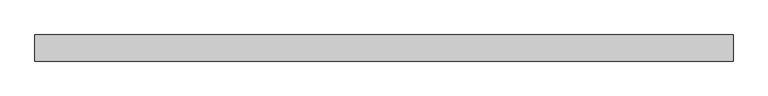
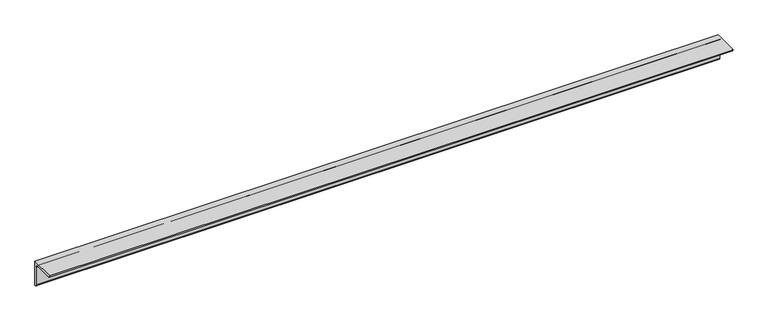
"""IFC4 building model written with IfcOpenShell, lengths in millimetres: member geometry, 0912_Steel Framing_L-KSD3502 : H_SB_AR_S03_L-130x130x12_HBR3."""

from ifc_helpers import new_model, si_unit, point, frame, frame_2d, origin, place, context, project, spatial, polyline, circle_curve, trimmed, segment, composite_curve, outline, extrude, source, transform, mapped, element, save


def member_96dd18ea(model_context):
    return source(origin(), model_context, "Body", "SweptSolid", [
        extrude(outline(composite_curve([segment(polyline([(36.4, 36.4), (36.4, -93.6)]), True, "CONTINUOUS"), segment(trimmed(circle_curve(frame_2d((36.4, -81.6)), 12.0), [point((36.4, -93.6))], [point((24.4, -81.6))], False, "CARTESIAN"), True, "CONTINUOUS"), segment(polyline([(24.4, -81.6), (24.4, 12.4)]), True, "CONTINUOUS"), segment(trimmed(circle_curve(frame_2d((12.4, 12.4)), 12.0), [point((24.4, 12.4))], [point((12.4, 24.4))], True, "CARTESIAN"), True, "CONTINUOUS"), segment(polyline([(12.4, 24.4), (-81.6, 24.4)]), True, "CONTINUOUS"), segment(trimmed(circle_curve(frame_2d((-81.6, 36.4)), 12.0), [point((-81.6, 24.4))], [point((-93.6, 36.4))], False, "CARTESIAN"), True, "CONTINUOUS"), segment(polyline([(-93.6, 36.4), (36.4, 36.4)]), True, "CONTINUOUS")], self_intersect=False)), frame((-1725.9882183, 0.0, 0.0), z_axis=(1.0, 0.0, 0.0), x_axis=(0.0, 1.0, 0.0)), (0.0, 0.0, 1.0), 3476.5545794),
    ])


if __name__ == "__main__":
    model = new_model("IFC4")
    model_context = context("Model", 3, world=origin())
    ifc_project = project(units=[si_unit("LENGTHUNIT", "METRE", prefix="MILLI")], contexts=[model_context])
    site = spatial("IfcSite", under=ifc_project)
    building = spatial("IfcBuilding", under=site)
    placement = place(None, origin())
    member_shape = member_96dd18ea(model_context)
    element("IfcMember", 1, ObjectType="0912_Steel Framing_L-KSD3502 : H_SB_AR_S03_L-130x130x12_HBR3", at=placement, inside=building, context=model_context, shape_type="MappedRepresentation", body=[
        mapped(member_shape, transform((0.0, 0.0, 0.0), x_axis=(1.0, 0.0, 0.0), y_axis=(0.0, 1.0, 0.0), z_axis=(0.0, 0.0, 1.0))),
    ])
    save(model, "model.ifc")

# Revit data of these elements
# Type "0912_Steel Framing_L-KSD3502 : H_SB_AR_S03_L-130x130x12_HBR3"
#   k = 25 mm
#   Perimeter = 0.52 m²/m
#   Nominal Weight = 23.40 kgf/m
#   Length [instance default] = 1000 mm
#   b = 130 mm
#   d = 130 mm
#   t = 12 mm
#   x = 36.4 mm
#   y = 36.4 mm
#   A = 2976.00 m²
#   Structural Material [instance default] = Steel, 45-345
# Element 1 (IfcMember, "0912_Steel Framing_L-KSD3502 : H_SB_AR_S03_L-130x130x12_HBR3")
#   Structural Material = Steel ASTM A36
#   Materials on its faces: "Steel ASTM A36"
# Materials
#   "Steel, 45-345": class "Metal", colour RGB 189 187 185, transparency 0, Description = "Steel 345 MPa", Cost = 0
#   "Steel ASTM A36": class "Metal", colour RGB 199 199 199, transparency 0, Description = "Structural steel, ASTM A36 Grade B, mill finish", Cost = 0
